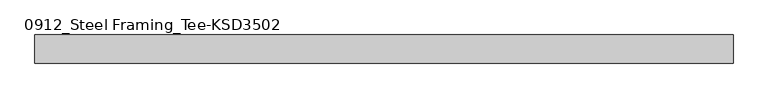
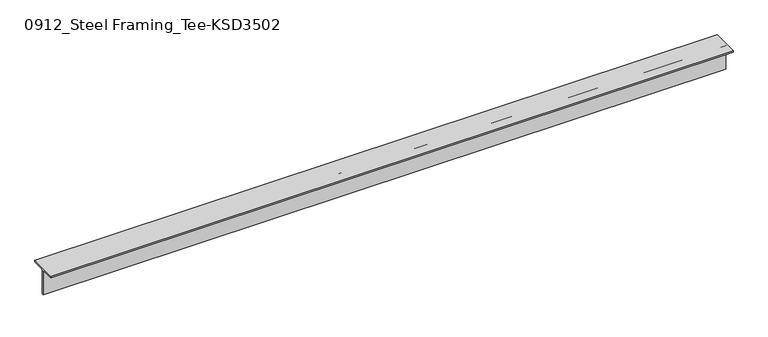
"""IFC4 building model written with IfcOpenShell, lengths in millimetres: member geometry, 0912_Steel Framing_Tee-KSD3502 : H_SB_ASB_CT-150x150x6.5x9."""

from ifc_helpers import new_model, si_unit, point, frame, frame_2d, origin, place, context, project, spatial, polyline, circle_curve, trimmed, segment, composite_curve, outline, extrude, source, transform, mapped, element, save


def member_0912_steel_framing_tee_ksd3502_8bc658f4(model_context):
    return source(origin(), model_context, "Body", "SweptSolid", [
        extrude(outline(composite_curve([segment(polyline([(-75.0, 75.0), (75.0, 75.0), (75.0, 66.0), (16.25, 66.0)]), True, "CONTINUOUS"), segment(trimmed(circle_curve(frame_2d((16.25, 53.0)), 13.0), [point((16.25, 66.0))], [point((3.25, 53.0))], True, "CARTESIAN"), True, "CONTINUOUS"), segment(polyline([(3.25, 53.0), (3.25, -75.0), (-3.25, -75.0), (-3.25, 53.0)]), True, "CONTINUOUS"), segment(trimmed(circle_curve(frame_2d((-16.25, 53.0)), 13.0), [point((-3.25, 53.0))], [point((-16.25, 66.0))], True, "CARTESIAN"), True, "CONTINUOUS"), segment(polyline([(-16.25, 66.0), (-75.0, 66.0), (-75.0, 75.0)]), True, "CONTINUOUS")], self_intersect=False)), frame((-1840.25, 0.0, 0.0), z_axis=(1.0, 0.0, 0.0), x_axis=(0.0, 1.0, 0.0)), (0.0, 0.0, 1.0), 3728.1),
    ])


if __name__ == "__main__":
    model = new_model("IFC4")
    model_context = context("Model", 3, world=origin())
    ifc_project = project(units=[si_unit("LENGTHUNIT", "METRE", prefix="MILLI")], contexts=[model_context])
    site = spatial("IfcSite", under=ifc_project)
    building = spatial("IfcBuilding", under=site)
    placement = place(None, origin())
    member_0912_steel_framing_tee_ksd3502_shape = member_0912_steel_framing_tee_ksd3502_8bc658f4(model_context)
    element("IfcMember", 1, ObjectType="0912_Steel Framing_Tee-KSD3502 : H_SB_ASB_CT-150x150x6.5x9", at=placement, inside=building, context=model_context, shape_type="MappedRepresentation", body=[
        mapped(member_0912_steel_framing_tee_ksd3502_shape, transform((0.0, 0.0, 0.0), x_axis=(1.0, 0.0, 0.0), y_axis=(0.0, 1.0, 0.0), z_axis=(0.0, 0.0, 1.0))),
    ])
    save(model, "model.ifc")

# Revit data of these elements
# Type "0912_Steel Framing_Tee-KSD3502 : H_SB_ASB_CT-150x150x6.5x9"
#   H_WM Code_1 = "S01AA003-00001 | Main Steel Structure Fabrication Work | Shelter/Building | Light Steel - Standard (30KG/M>Weight) | Material: (   )"
#   H_WM Code_2 = "S03AA029-00001 | Main Steel Structure Erection Work | Shelter/Building | Light Steel (30KG/M>Weight) | Material: (   )"
#   H_WM Code_3 = "S01AA010-00001 | Main Steel Structure Fabrication Work | Shelter/Building | Steel Painting/Coating | for Non-Fireproofed Steel Surface, Surface Preparation, Primer, Second & Final Coat | Material: (   )"
#   H_Q'ty Cal Type Tag = "SB-Q2"
#   Width = 15.0 cm
#   Web Thickness = 0.65 cm
#   Web Fillet = 1.3 cm
#   Section Area = 23.39 cm²
#   Perimeter = 0.60 m²/m
#   Nominal Weight = 18.40 kgf/m
#   Height = 15.0 cm
#   Flange Thickness = 0.9 cm
#   Centroid Vertical = 7.5 cm
#   Centroid Horizontal = 7.5 cm
#   Length [instance default] = 1.5000 m
#   Structural Material [instance default] = Steel, 45-345
#   Warping Constant = (empty or 0)
#   Torsional Moment of Inertia = 0
#   Section Name Key = ""
#   Plastic Modulus weak axis = 0
#   Plastic Modulus strong axis = 0
#   Moment of Inertia weak axis = 0
#   Moment of Inertia strong axis = 0
#   Elastic Modulus weak axis = 0
#   Elastic Modulus strong axis = 0
#   Bolt Spacing = 0
#   Assembly Code = ""
# Element 1 (IfcMember, "0912_Steel Framing_Tee-KSD3502 : H_SB_ASB_CT-150x150x6.5x9")
#   Structural Material = none
# Materials
#   "Steel, 45-345": class "Metal", colour RGB 189 187 185, transparency 0, Description = "Steel 345 MPa", Cost = 0
